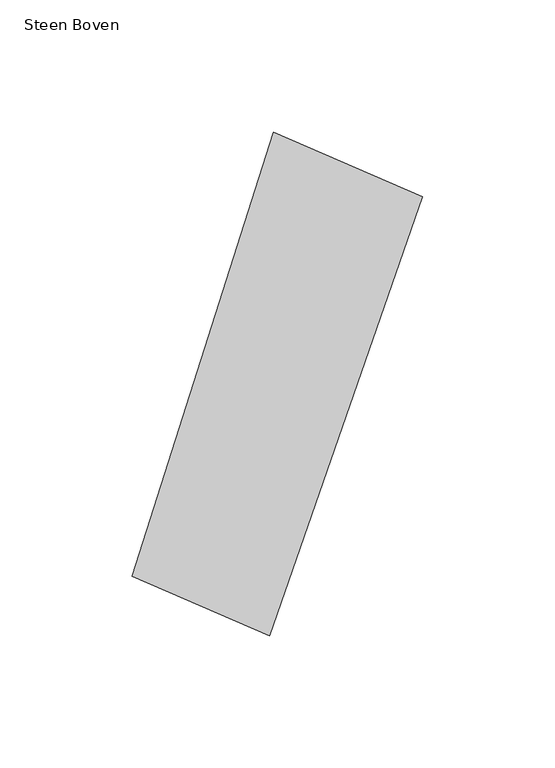
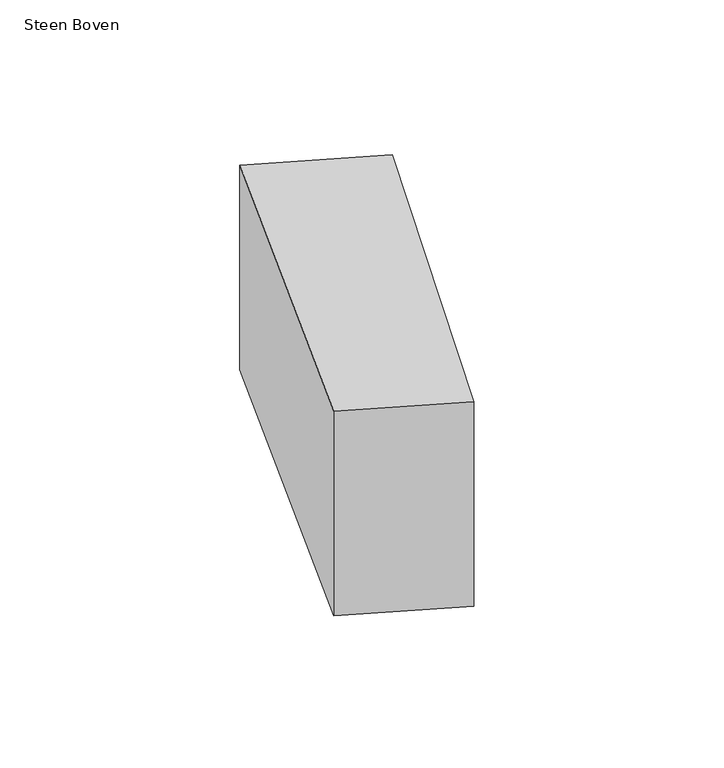
"""IFC4 building model written with IfcOpenShell, lengths in millimetres: proxy geometry, 00_GMA_steen_versie_4 : Steen Boven."""

from ifc_helpers import new_model, si_unit, origin, origin_with_axes, place, context, project, spatial, polyline, outline, extrude, source, transform, mapped, element, save


def steen_boven_f08e2b57(model_context):
    return source(origin(), model_context, "Body", "SweptSolid", [
        extrude(outline(polyline([(130.7380398, 155.7532406), (72.8371145, -9.8774388), (21.0289728, 12.481511), (74.3421688, 180.1043212), (130.7380398, 155.7532406)])), origin_with_axes(), (0.0, 0.0, 1.0), 100.0),
    ])


if __name__ == "__main__":
    model = new_model("IFC4")
    model_context = context("Model", 3, world=origin())
    ifc_project = project(units=[si_unit("LENGTHUNIT", "METRE", prefix="MILLI")], contexts=[model_context])
    site = spatial("IfcSite", under=ifc_project)
    building = spatial("IfcBuilding", under=site)
    placement = place(None, origin())
    steen_boven_shape = steen_boven_f08e2b57(model_context)
    element("IfcBuildingElementProxy", 1, Name="00_GMA_steen_versie_4 : Steen Boven", ObjectType="00_GMA_steen_versie_4 : Steen Boven", at=placement, inside=building, context=model_context, shape_type="MappedRepresentation", body=[
        mapped(steen_boven_shape, transform((0.0, 0.0, 0.0), x_axis=(1.0, 0.0, 0.0), y_axis=(0.0, 1.0, 0.0), z_axis=(0.0, 0.0, 1.0))),
    ])
    save(model, "model.ifc")

# Revit data of these elements
# Type "00_GMA_steen_versie_4 : Steen Boven"
#   StootVoegHalfBoven [instance default] = 5 mm
#   StootVoegHalf [instance default] = 5 mm
#   StootVoegBreedteOnder = 10 mm
#   StootVoegBreedteBoven = 10 mm
#   Steendikte = 100 mm
#   LintVoegOnderHalf = 5 mm
#   LintVoegOnder = 10 mm
#   LintVoegBovenHalf = 0 mm
#   LintVoegBoven = 0 mm
#   materiaal = none
#   MateriaalVoeg = none
#   Default Elevation = 0
